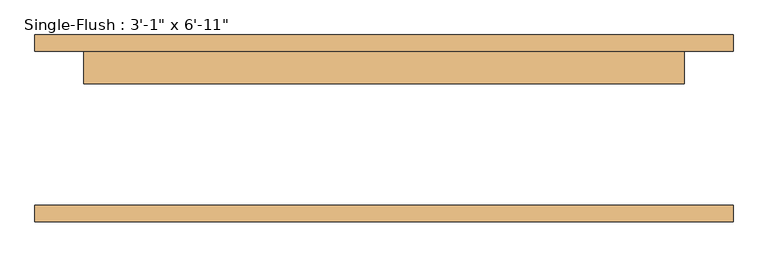
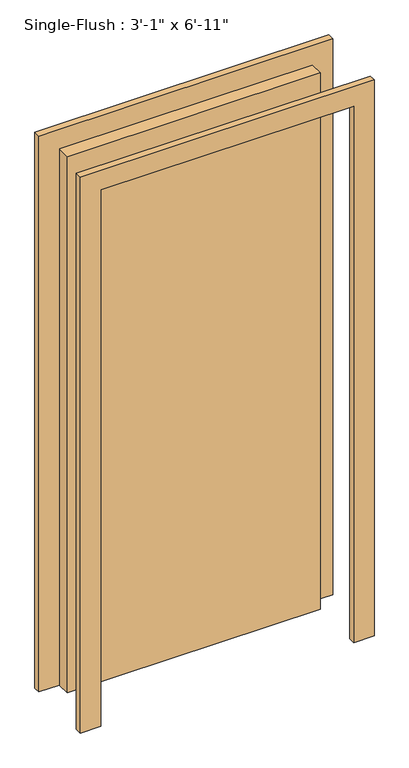
"""IFC4 building model written with IfcOpenShell, lengths in millimetres: door geometry."""

from ifc_helpers import new_model, si_unit, frame, origin, origin_with_axes, place, context, project, spatial, polyline, outline, extrude, source, transform, mapped, element, save


def door_4a887283(model_context):
    return source(origin(), model_context, "Body", "SweptSolid", [
        extrude(outline(polyline([(2184.4, -546.1), (0.0, -546.1), (0.0, -469.9), (2108.2, -469.9), (2108.2, 469.9), (0.0, 469.9), (0.0, 546.1), (2184.4, 546.1), (2184.4, -546.1)])), frame((0.0, 120.65, 0.0), z_axis=(0.0, 1.0, 0.0), x_axis=(0.0, 0.0, 1.0)), (0.0, 0.0, 1.0), 25.4),
        extrude(outline(polyline([(2184.4, 546.1), (2184.4, -546.1), (0.0, -546.1), (0.0, -469.9), (2108.2, -469.9), (2108.2, 469.9), (0.0, 469.9), (0.0, 546.1), (2184.4, 546.1)])), frame((0.0, -146.05, 0.0), z_axis=(0.0, 1.0, 0.0), x_axis=(0.0, 0.0, 1.0)), (0.0, 0.0, 1.0), 25.4),
        extrude(outline(polyline([(469.9, 69.85), (-469.9, 69.85), (-469.9, 120.65), (469.9, 120.65), (469.9, 69.85)])), origin_with_axes(), (0.0, 0.0, 1.0), 2108.2),
    ])


if __name__ == "__main__":
    model = new_model("IFC4")
    model_context = context("Model", 3, world=origin())
    ifc_project = project(units=[si_unit("LENGTHUNIT", "METRE", prefix="MILLI")], contexts=[model_context])
    site = spatial("IfcSite", under=ifc_project)
    building = spatial("IfcBuilding", under=site)
    placement = place(None, origin())
    door_shape = door_4a887283(model_context)
    element("IfcDoor", 1, ObjectType="Single-Flush : 3'-1\" x 6'-11\"", at=placement, inside=building, context=model_context, shape_type="MappedRepresentation", body=[
        mapped(door_shape, transform((0.0, 0.0, 0.0), x_axis=(1.0, 0.0, 0.0), y_axis=(0.0, 1.0, 0.0), z_axis=(0.0, 0.0, 1.0))),
    ])
    save(model, "model.ifc")

# Revit data of these elements
# Type "Single-Flush : 3'-1\" x 6'-11\""
#   Type Mark = "17"
#   Construction Type Id = "MDOOR"
#   Assembly Code = "C1020"
#   Analytic Construction = "Metal"
#   Thickness = 0' - 2"
#   Heat Transfer Coefficient (U) = 3.7021 W/(m²·K)
#   Height = 6' - 11"
#   Trim Projection Ext = 0' - 1"
#   Trim Projection Int = 0' - 1"
#   Trim Width = 0' - 3"
#   Width = 3' - 1"
#   Door Material = Door - Panel
#   Frame Material = Door - Frame
#   Visual Light Transmittance = 0
#   Solar Heat Gain Coefficient = 0
#   Function = (empty or 0)
#   Wall Closure = (empty or 0)
# Element 1 (IfcDoor, "Single-Flush : 3'-1\" x 6'-11\"")
#   Materials on its faces: "Door - Frame", "Door - Panel"
# Materials
#   "Door - Panel": class "Wood", colour RGB 210 159 95, transparency 0, Cost = 0
#   "Door - Frame": class "Miscellaneous", colour RGB 118 70 51, transparency 0, Cost = 0
